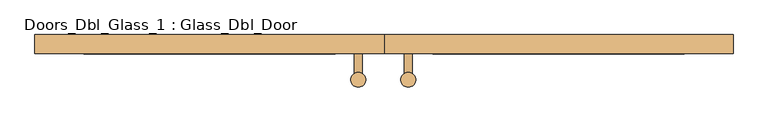
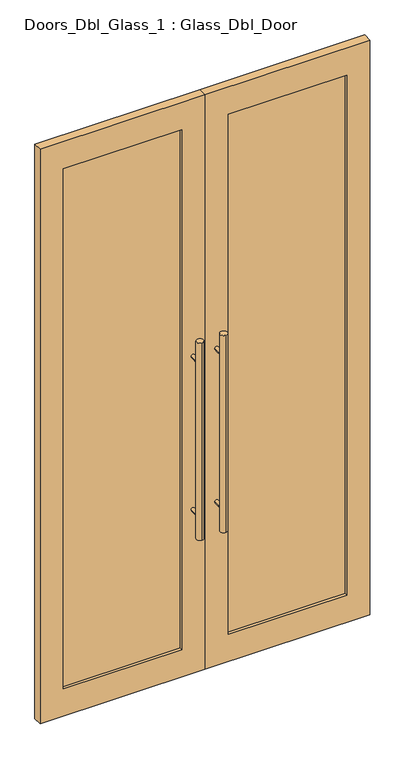
"""IFC4 building model written with IfcOpenShell, lengths in millimetres: door geometry, Doors_Dbl_Glass_1 : Glass_Dbl_Door."""

from ifc_helpers import new_model, si_unit, point, frame, frame_2d, origin, place, context, project, spatial, polyline, circle_curve, trimmed, segment, composite_curve, outline, extrude, source, transform, mapped, element, save


def doors_dbl_glass_1_glass_dbl_door_233ab62a(model_context):
    return source(origin(), model_context, "Body", "SweptSolid", [
        extrude(outline(composite_curve([segment(trimmed(circle_curve(frame_2d((49.6069979, -116.0715804)), 15.0), [point((49.6069979, -101.0715804))], [point((49.6069979, -131.0715804))], False, "CARTESIAN"), True, "CONTINUOUS"), segment(trimmed(circle_curve(frame_2d((49.6069979, -116.0715804)), 15.0), [point((49.6069979, -131.0715804))], [point((49.6069979, -101.0715804))], False, "CARTESIAN"), True, "CONTINUOUS")], self_intersect=False)), frame((0.0, 0.0, 650.0), z_axis=(0.0, 0.0, 1.0), x_axis=(1.0, 0.0, 0.0)), (0.0, 0.0, 1.0), 900.0),
        extrude(outline(composite_curve([segment(trimmed(circle_curve(frame_2d((-52.537897, -116.0715804)), 15.0), [point((-52.537897, -101.0715804))], [point((-52.537897, -131.0715804))], False, "CARTESIAN"), True, "CONTINUOUS"), segment(trimmed(circle_curve(frame_2d((-52.537897, -116.0715804)), 15.0), [point((-52.537897, -131.0715804))], [point((-52.537897, -101.0715804))], False, "CARTESIAN"), True, "CONTINUOUS")], self_intersect=False)), frame((0.0, 0.0, 650.0), z_axis=(0.0, 0.0, 1.0), x_axis=(1.0, 0.0, 0.0)), (0.0, 0.0, 1.0), 900.0),
        extrude(outline(composite_curve([segment(trimmed(circle_curve(frame_2d((750.0, 49.6069979)), 8.0), [point((750.0, 57.6069979))], [point((750.0, 41.6069979))], False, "CARTESIAN"), True, "CONTINUOUS"), segment(trimmed(circle_curve(frame_2d((750.0, 49.6069979)), 8.0), [point((750.0, 41.6069979))], [point((750.0, 57.6069979))], False, "CARTESIAN"), True, "CONTINUOUS")], self_intersect=False)), frame((0.0, -116.0715804, 0.0), z_axis=(0.0, 1.0, 0.0), x_axis=(0.0, 0.0, 1.0)), (0.0, 0.0, 1.0), 53.4927248),
        extrude(outline(composite_curve([segment(trimmed(circle_curve(frame_2d((750.0, -52.537897)), 8.0), [point((750.0, -44.537897))], [point((750.0, -60.537897))], False, "CARTESIAN"), True, "CONTINUOUS"), segment(trimmed(circle_curve(frame_2d((750.0, -52.537897)), 8.0), [point((750.0, -60.537897))], [point((750.0, -44.537897))], False, "CARTESIAN"), True, "CONTINUOUS")], self_intersect=False)), frame((0.0, -116.0715804, 0.0), z_axis=(0.0, 1.0, 0.0), x_axis=(0.0, 0.0, 1.0)), (0.0, 0.0, 1.0), 53.4927248),
        extrude(outline(composite_curve([segment(trimmed(circle_curve(frame_2d((1450.0, 49.6069979)), 8.0), [point((1450.0, 57.6069979))], [point((1450.0, 41.6069979))], False, "CARTESIAN"), True, "CONTINUOUS"), segment(trimmed(circle_curve(frame_2d((1450.0, 49.6069979)), 8.0), [point((1450.0, 41.6069979))], [point((1450.0, 57.6069979))], False, "CARTESIAN"), True, "CONTINUOUS")], self_intersect=False)), frame((0.0, -116.0715804, 0.0), z_axis=(0.0, 1.0, 0.0), x_axis=(0.0, 0.0, 1.0)), (0.0, 0.0, 1.0), 53.4927248),
        extrude(outline(composite_curve([segment(trimmed(circle_curve(frame_2d((1450.0, -52.537897)), 8.0), [point((1450.0, -44.537897))], [point((1450.0, -60.537897))], False, "CARTESIAN"), True, "CONTINUOUS"), segment(trimmed(circle_curve(frame_2d((1450.0, -52.537897)), 8.0), [point((1450.0, -60.537897))], [point((1450.0, -44.537897))], False, "CARTESIAN"), True, "CONTINUOUS")], self_intersect=False)), frame((0.0, -116.0715804, 0.0), z_axis=(0.0, 1.0, 0.0), x_axis=(0.0, 0.0, 1.0)), (0.0, 0.0, 1.0), 53.4927248),
        extrude(outline(polyline([(2625.0, -712.5), (0.0, -712.5), (0.0, 0.0), (2625.0, 0.0), (2625.0, -712.5)]), holes=[polyline([(2500.0, -612.5), (2500.0, -100.0), (125.0, -100.0), (125.0, -612.5), (2500.0, -612.5)])]), frame((0.0, -62.5788556, 0.0), z_axis=(0.0, 1.0, 0.0), x_axis=(0.0, 0.0, 1.0)), (0.0, 0.0, 1.0), 38.5435966),
        extrude(outline(polyline([(2625.0, 0.0), (0.0, 0.0), (0.0, 712.5), (2625.0, 712.5), (2625.0, 0.0)]), holes=[polyline([(2500.0, 100.0), (2500.0, 612.5), (125.0, 612.5), (125.0, 100.0), (2500.0, 100.0)])]), frame((0.0, -62.5788556, 0.0), z_axis=(0.0, 1.0, 0.0), x_axis=(0.0, 0.0, 1.0)), (0.0, 0.0, 1.0), 38.5435966),
        extrude(outline(polyline([(-100.0, -38.0), (-100.0, -50.0), (-612.5, -50.0), (-612.5, -38.0), (-100.0, -38.0)])), frame((0.0, 0.0, 125.0), z_axis=(0.0, 0.0, 1.0), x_axis=(1.0, 0.0, 0.0)), (0.0, 0.0, 1.0), 2375.0),
        extrude(outline(polyline([(612.5, -38.0), (612.5, -50.0), (100.0, -50.0), (100.0, -38.0), (612.5, -38.0)])), frame((0.0, 0.0, 125.0), z_axis=(0.0, 0.0, 1.0), x_axis=(1.0, 0.0, 0.0)), (0.0, 0.0, 1.0), 2375.0),
    ])


if __name__ == "__main__":
    model = new_model("IFC4")
    model_context = context("Model", 3, world=origin())
    ifc_project = project(units=[si_unit("LENGTHUNIT", "METRE", prefix="MILLI")], contexts=[model_context])
    site = spatial("IfcSite", under=ifc_project)
    building = spatial("IfcBuilding", under=site)
    placement = place(None, origin())
    doors_dbl_glass_1_glass_dbl_door_shape = doors_dbl_glass_1_glass_dbl_door_233ab62a(model_context)
    element("IfcDoor", 1, ObjectType="Doors_Dbl_Glass_1 : Glass_Dbl_Door", at=placement, inside=building, context=model_context, shape_type="MappedRepresentation", body=[
        mapped(doors_dbl_glass_1_glass_dbl_door_shape, transform((0.0, 0.0, 0.0), x_axis=(1.0, 0.0, 0.0), y_axis=(0.0, 1.0, 0.0), z_axis=(0.0, 0.0, 1.0))),
    ])
    save(model, "model.ifc")

# Revit data of these elements
# Type "Doors_Dbl_Glass_1 : Glass_Dbl_Door"
#   Type Mark = "48"
#   Construction Type Id = "GSP4R"
#   Analytic Construction = "1/8 in Pilkington single glazing"
#   Visual Light Transmittance = 0.9
#   Stile Shutting = 100 mm
#   Stile Hanging = 100 mm
#   Stile - Top Rail = 125 mm
#   Stile - Bottom Rail = 125 mm
#   Solar Heat Gain Coefficient = 0.78
#   Offset = 50 mm
#   Heat Transfer Coefficient (U) = 3.6886 W/(m²·K)
#   Glass Thickness = 12 mm
#   Define Thermal Properties by = 1
#   Material Ironmongery = Metal - Aluminum
#   Material Door = Metal - Aluminum
#   Material Glass = Glass
#   Function = (empty or 0)
# Element 1 (IfcDoor, "Doors_Dbl_Glass_1 : Glass_Dbl_Door")
#   Materials on its faces: "Metal - Aluminum", "Glass"
# Materials
#   "Metal - Aluminum": class "Metal", colour RGB 247 247 247, transparency 0
#   "Glass": class "Glass", colour RGB 0 128 192, transparency 0.9, Description = "Soda Lime Glass", Cost = 0
